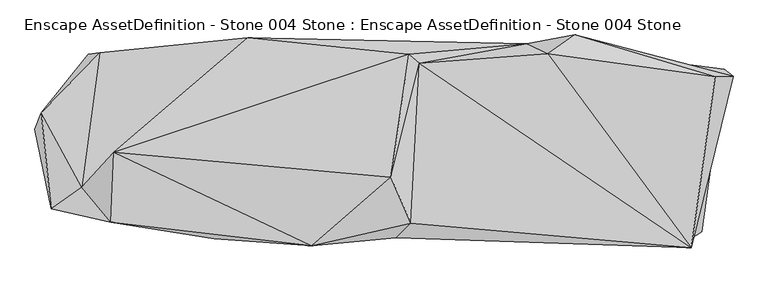
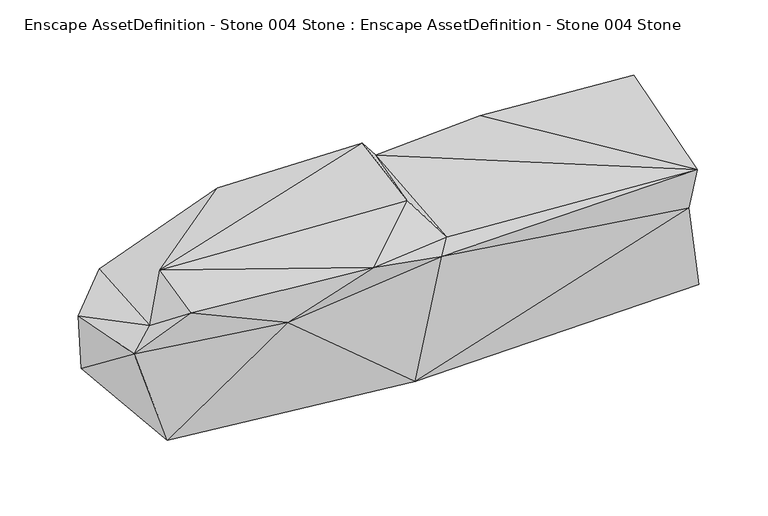
"""IFC4 building model written with IfcOpenShell, lengths in millimetres: geographic element geometry, Enscape AssetDefinition - Stone 004 Stone : Enscape AssetDefinition - Stone 004 Stone."""

from ifc_helpers import new_model, si_unit, origin, place, context, project, spatial, faceted_brep, source, transform, mapped, element, save


def enscape_assetdefinition_stone_004_stone_enscape_63bbff13(model_context):
    return source(origin(), model_context, "Body", "Brep", [
        faceted_brep([(-38.9318503, -164.1649306, -1.7086391), (576.9498348, -158.3960354, 1.3118839), (543.9553261, -179.3752164, 199.9496669), (617.8355217, 140.3366923, 1.3128809), (255.6339502, 187.2245818, 0.647967), (634.4404221, 127.5458336, 206.1242908), (15.7774985, -169.4483608, 268.6451375), (557.3483109, -187.6831353, 287.8977358), (343.3826566, 203.5553306, 247.4047691), (601.2535691, 126.5848428, 298.6131012), (294.178009, 168.8552201, 288.1190479), (57.723891, 151.101917, 291.0897136), (41.9543684, -142.6275074, 287.3643935), (5.2156355, -58.0169708, 332.1199715), (38.5121666, 167.9949164, 315.0704503), (-139.4893527, -184.065491, 306.1634004), (-503.415525, -12.3193478, 323.6864209), (-257.1521997, 198.1841922, 297.6062596), (-562.1462464, -76.3444677, 256.3566566), (-508.8983178, -140.8132017, 304.8056662), (-318.6931014, -171.0244119, 235.8121425), (-618.8135147, -116.2233427, 234.839201), (-528.947413, 170.5508977, 224.4617492), (-636.7661357, 60.6586821, 221.505031), (-550.0053167, -121.8566746, 17.1561725), (-648.4425068, 30.5032954, 123.7836331), (-566.0041571, 93.6561599, 100.8236632), (-427.8805256, 176.4503866, 1.5531271), (-550.8586764, 167.8623408, 142.3653215)], [[[0, 1, 2]], [[2, 1, 3]], [[0, 4, 1]], [[1, 4, 3]], [[5, 2, 3]], [[6, 0, 2]], [[2, 7, 6]], [[5, 7, 2]], [[5, 3, 4]], [[8, 5, 4]], [[5, 8, 9]], [[7, 5, 9]], [[10, 11, 7]], [[12, 7, 11]], [[10, 7, 9]], [[12, 6, 7]], [[8, 10, 9]], [[10, 8, 4]], [[11, 10, 4]], [[11, 13, 12]], [[14, 13, 11]], [[11, 4, 14]], [[15, 12, 13]], [[15, 6, 12]], [[14, 16, 13]], [[15, 13, 16]], [[17, 14, 4]], [[16, 14, 17]], [[16, 17, 18]], [[19, 15, 16]], [[16, 18, 19]], [[19, 20, 15]], [[6, 15, 20]], [[20, 19, 21]], [[18, 21, 19]], [[18, 22, 23]], [[23, 21, 18]], [[17, 22, 18]], [[24, 20, 21]], [[23, 25, 21]], [[25, 24, 21]], [[0, 6, 20]], [[24, 0, 20]], [[25, 26, 24]], [[0, 24, 27]], [[26, 27, 24]], [[26, 25, 23]], [[22, 28, 23]], [[28, 26, 23]], [[22, 17, 28]], [[17, 27, 28]], [[26, 28, 27]], [[27, 17, 4]], [[27, 4, 0]]]),
    ])


if __name__ == "__main__":
    model = new_model("IFC4")
    model_context = context("Model", 3, world=origin())
    ifc_project = project(units=[si_unit("LENGTHUNIT", "METRE", prefix="MILLI")], contexts=[model_context])
    site = spatial("IfcSite", under=ifc_project)
    building = spatial("IfcBuilding", under=site)
    placement = place(None, origin())
    enscape_assetdefinition_stone_004_stone_enscape_shape = enscape_assetdefinition_stone_004_stone_enscape_63bbff13(model_context)
    element("IfcGeographicElement", 1, ObjectType="Enscape AssetDefinition - Stone 004 Stone : Enscape AssetDefinition - Stone 004 Stone", at=placement, inside=building, context=model_context, shape_type="MappedRepresentation", body=[
        mapped(enscape_assetdefinition_stone_004_stone_enscape_shape, transform((0.0, 0.0, 0.0), x_axis=(1.0, 0.0, 0.0), y_axis=(0.0, 1.0, 0.0), z_axis=(0.0, 0.0, 1.0))),
    ])
    save(model, "model.ifc")

# Revit data of these elements
# Type "Enscape AssetDefinition - Stone 004 Stone : Enscape AssetDefinition - Stone 004 Stone"
#   EnscapeAssetSource = "REMOTE"
#   EnscapeAssetId = "ab028e80-cffe-4f02-88c2-ad31a551f3f6"
#   Height = 0.33212 m
#   EnscapeNativeAssetHeight = 0.33212 m
#   Default Elevation = 0
